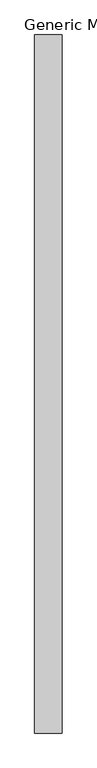
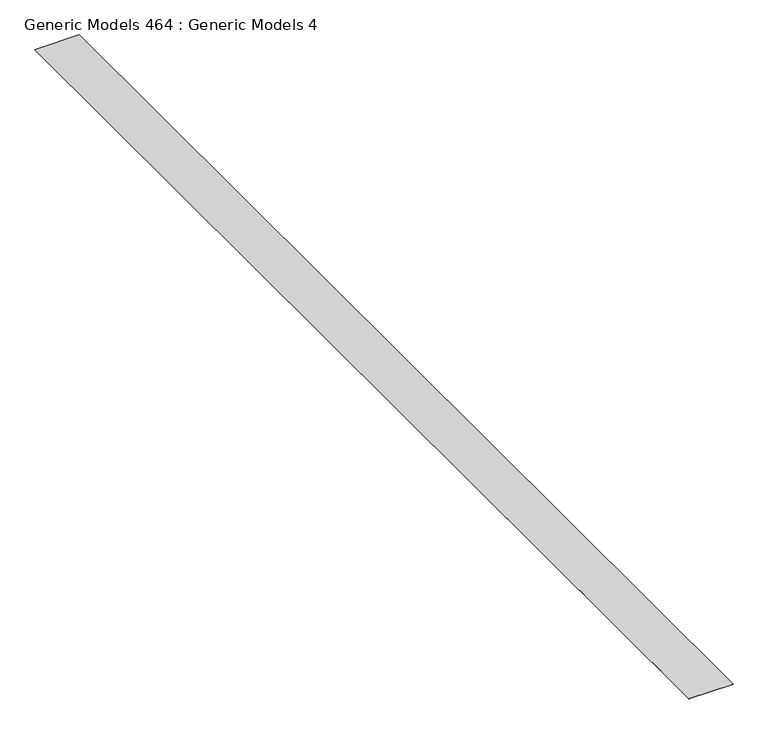
"""IFC4 building model written with IfcOpenShell, lengths in millimetres: proxy geometry, Generic Models 464 : Generic Models 4."""

from ifc_helpers import new_model, si_unit, frame, origin, place, context, project, spatial, polyline, outline, extrude, source, transform, mapped, element, save


def generic_models_464_generic_models_4_2895484c(model_context):
    return source(origin(), model_context, "Body", "SweptSolid", [
        extrude(outline(polyline([(1422.2263704, -5493.3230338), (933.2763704, -5493.3230338), (933.2763704, 7054.2769662), (1422.2263704, 7054.2769662), (1422.2263704, -5493.3230338)])), frame((0.0, 0.0, 123180.221), z_axis=(0.0, 0.0, 1.0), x_axis=(1.0, 0.0, 0.0)), (0.0, 0.0, 1.0), 1.5875),
    ])


if __name__ == "__main__":
    model = new_model("IFC4")
    model_context = context("Model", 3, world=origin())
    ifc_project = project(units=[si_unit("LENGTHUNIT", "METRE", prefix="MILLI")], contexts=[model_context])
    site = spatial("IfcSite", under=ifc_project)
    building = spatial("IfcBuilding", under=site)
    placement = place(None, origin())
    generic_models_464_generic_models_4_shape = generic_models_464_generic_models_4_2895484c(model_context)
    element("IfcBuildingElementProxy", 1, Name="Generic Models 464 : Generic Models 4", ObjectType="Generic Models 464 : Generic Models 4", at=placement, inside=building, context=model_context, shape_type="MappedRepresentation", body=[
        mapped(generic_models_464_generic_models_4_shape, transform((0.0, 0.0, 0.0), x_axis=(1.0, 0.0, 0.0), y_axis=(0.0, 1.0, 0.0), z_axis=(0.0, 0.0, 1.0))),
    ])
    save(model, "model.ifc")

# Revit data of these elements
# Element 1 (IfcBuildingElementProxy, "Generic Models 464 : Generic Models 4")
#   Materials on its faces: "_15 MIL VAPOR BARRIER"
# Materials
#   "_15 MIL VAPOR BARRIER": class "Generic", colour RGB 67 154 161, transparency 0, Cost = 0
